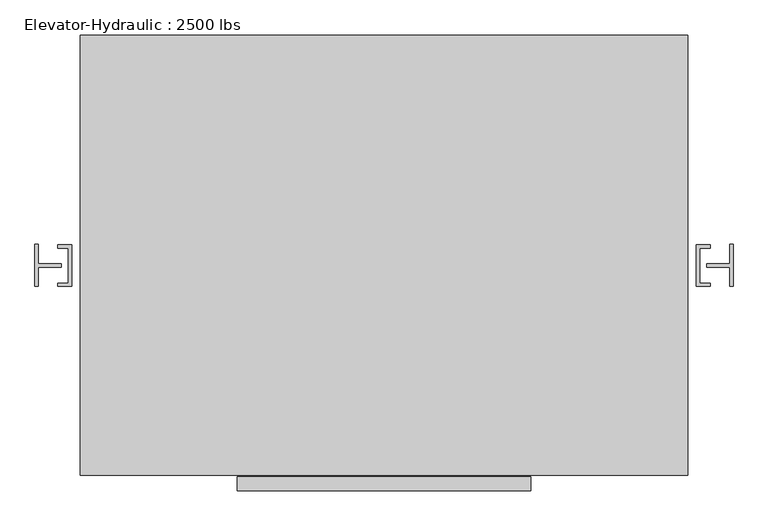
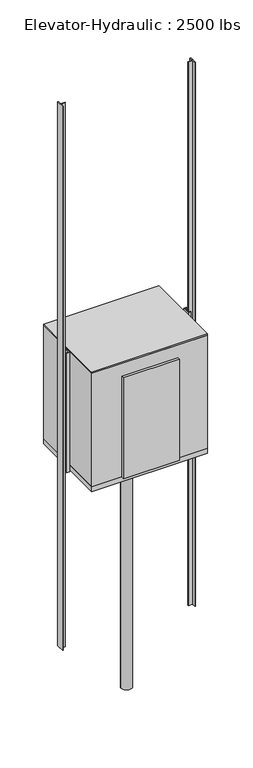
"""IFC4 building model written with IfcOpenShell, lengths in millimetres: proxy geometry, Elevator-Hydraulic : 2500 lbs."""

from ifc_helpers import new_model, si_unit, point, frame, frame_2d, origin, origin_with_axes, place, context, project, spatial, polyline, circle_curve, trimmed, segment, composite_curve, outline, extrude, faceted_brep, source, transform, mapped, element, save


def elevator_hydraulic_2500_lbs_0286828a(model_context):
    return source(origin(), model_context, "Body", "SolidModel", [
        extrude(outline(polyline([(540.8469965, -765.5281737), (540.8469965, -816.3281737), (-525.9530035, -816.3281737), (-525.9530035, -765.5281737), (540.8469965, -765.5281737)])), frame((0.0, 0.0, 3657.6), z_axis=(0.0, 0.0, 1.0), x_axis=(1.0, 0.0, 0.0)), (0.0, 0.0, 1.0), 2032.0),
        extrude(outline(polyline([(1112.3469965, 841.0218263), (1112.3469965, -759.1781737), (-1097.4530035, -759.1781737), (-1097.4530035, 841.0218263), (1112.3469965, 841.0218263)])), frame((0.0, 0.0, 5943.6), z_axis=(0.0, 0.0, 1.0), x_axis=(1.0, 0.0, 0.0)), (0.0, 0.0, 1.0), 25.4),
        extrude(outline(composite_curve([segment(trimmed(circle_curve(frame_2d((7.4469965, 2.8218263)), 101.6), [point((-94.1530035, 2.8218263))], [point((109.0469965, 2.8218263))], False, "CARTESIAN"), True, "CONTINUOUS"), segment(trimmed(circle_curve(frame_2d((7.4469965, 2.8218263)), 101.6), [point((109.0469965, 2.8218263))], [point((-94.1530035, 2.8218263))], False, "CARTESIAN"), True, "CONTINUOUS")], self_intersect=False)), frame((0.0, 0.0, -1219.2), z_axis=(0.0, 0.0, 1.0), x_axis=(1.0, 0.0, 0.0)), (0.0, 0.0, 1.0), 4775.2),
        faceted_brep([(1112.3469965, 841.0218263, 5943.6), (-1097.4530035, 841.0218263, 5943.6), (-1097.4530035, -759.1781737, 5943.6), (1112.3469965, -759.1781737, 5943.6), (1074.2469965, 802.9218263, 5943.6), (1074.2469965, -721.0781737, 5943.6), (-1059.3530035, -721.0781737, 5943.6), (-1059.3530035, 802.9218263, 5943.6), (1074.2469965, 802.9218263, 3657.6), (-1059.3530035, 802.9218263, 3657.6), (-1059.3530035, -721.0781737, 3657.6), (-525.9530035, -721.0781737, 3657.6), (-525.9530035, -759.1781737, 3657.6), (-1097.4530035, -759.1781737, 3657.6), (-1097.4530035, 841.0218263, 3657.6), (1112.3469965, 841.0218263, 3657.6), (1112.3469965, -759.1781737, 3657.6), (540.8469965, -759.1781737, 3657.6), (540.8469965, -721.0781737, 3657.6), (1074.2469965, -721.0781737, 3657.6), (540.8469965, -721.0781737, 5689.6), (-525.9530035, -721.0781737, 5689.6), (-525.9530035, -759.1781737, 5689.6), (540.8469965, -759.1781737, 5689.6)], [[[0, 1, 2, 3], [4, 5, 6, 7]], [[8, 9, 10, 11, 12, 13, 14, 15, 16, 17, 18, 19]], [[5, 4, 8, 19]], [[6, 5, 19, 18, 20, 21, 11, 10]], [[7, 6, 10, 9]], [[4, 7, 9, 8]], [[1, 0, 15, 14]], [[2, 1, 14, 13]], [[3, 2, 13, 12, 22, 23, 17, 16]], [[0, 3, 16, 15]], [[22, 21, 20, 23]], [[21, 22, 12, 11]], [[23, 20, 18, 17]]]),
        extrude(outline(polyline([(1112.3469965, 841.0218263), (1112.3469965, -759.1781737), (-1097.4530035, -759.1781737), (-1097.4530035, 841.0218263), (1112.3469965, 841.0218263)])), frame((0.0, 0.0, 3556.0), z_axis=(0.0, 0.0, 1.0), x_axis=(1.0, 0.0, 0.0)), (0.0, 0.0, 1.0), 101.6),
        extrude(outline(polyline([(-1129.2030035, 79.0218263), (-1129.2030035, -73.3781737), (-1180.0030035, -73.3781737), (-1180.0030035, -60.6781737), (-1141.9030035, -60.6781737), (-1141.9030035, 66.3218263), (-1180.0030035, 66.3218263), (-1180.0030035, 79.0218263), (-1129.2030035, 79.0218263)])), frame((0.0, 0.0, 3556.0), z_axis=(0.0, 0.0, 1.0), x_axis=(1.0, 0.0, 0.0)), (0.0, 0.0, 1.0), 2413.0),
        extrude(outline(polyline([(1144.0969965, 79.0218263), (1194.8969965, 79.0218263), (1194.8969965, 66.3218263), (1156.7969965, 66.3218263), (1156.7969965, -60.6781737), (1194.8969965, -60.6781737), (1194.8969965, -73.3781737), (1144.0969965, -73.3781737), (1144.0969965, 79.0218263)])), frame((0.0, 0.0, 3556.0), z_axis=(0.0, 0.0, 1.0), x_axis=(1.0, 0.0, 0.0)), (0.0, 0.0, 1.0), 2413.0),
        extrude(outline(polyline([(-1249.8530035, 79.0218263), (-1249.8530035, 9.1718263), (-1167.3030035, 9.1718263), (-1167.3030035, -3.5281737), (-1249.8530035, -3.5281737), (-1249.8530035, -73.3781737), (-1262.5530035, -73.3781737), (-1262.5530035, 79.0218263), (-1249.8530035, 79.0218263)])), origin_with_axes(), (0.0, 0.0, 1.0), 10972.8),
        extrude(outline(polyline([(1264.7469965, 79.0218263), (1277.4469965, 79.0218263), (1277.4469965, -73.3781737), (1264.7469965, -73.3781737), (1264.7469965, -3.5281737), (1182.1969965, -3.5281737), (1182.1969965, 9.1718263), (1264.7469965, 9.1718263), (1264.7469965, 79.0218263)])), origin_with_axes(), (0.0, 0.0, 1.0), 10972.8),
    ])


if __name__ == "__main__":
    model = new_model("IFC4")
    model_context = context("Model", 3, world=origin())
    ifc_project = project(units=[si_unit("LENGTHUNIT", "METRE", prefix="MILLI")], contexts=[model_context])
    site = spatial("IfcSite", under=ifc_project)
    building = spatial("IfcBuilding", under=site)
    placement = place(None, origin())
    elevator_hydraulic_2500_lbs_shape = elevator_hydraulic_2500_lbs_0286828a(model_context)
    element("IfcBuildingElementProxy", 1, Name="Elevator-Hydraulic : 2500 lbs", ObjectType="Elevator-Hydraulic : 2500 lbs", at=placement, inside=building, context=model_context, shape_type="MappedRepresentation", body=[
        mapped(elevator_hydraulic_2500_lbs_shape, transform((0.0, 0.0, 0.0), x_axis=(1.0, 0.0, 0.0), y_axis=(0.0, 1.0, 0.0), z_axis=(0.0, 0.0, 1.0))),
    ])
    save(model, "model.ifc")

# Revit data of these elements
# Project information
#   Organization Name = "G3B Press"
#   Organization Description = "Paul F. Aubin Cosulting Services, Inc."
#   Building Name = "Revit Essentials for Architecture"
#   Author = "Paul F. Aubin"
#   Author Website = "https://www.paulaubin.com"
#   Copyright = "Copyright © 2020 Paul F Aubin, all rights reserved"
#   Project Issue Date = "8/1/2020"
#   Project Status = "Design Development"
#   Client Name = "Groups and Links"
#   Project Address = "Enter address here"
#   Project Name = "Hotel"
#   Project Number = "2020.06A"
# Type "Elevator-Hydraulic : 2500 lbs"
#   Cab Location = 12' - 0"
#   Width = 8' - 4"
#   Pit Depth = 4' - 0"
#   Height [instance default] = 36' - 0"
#   Door Opening = 3' - 6"
#   Depth = 5' - 9"
#   Cab Width = 7' - 0"
#   Cab Height = 7' - 6"
#   Cab Depth = 5' - 0"
#   Default Elevation = 0
# Element 1 (IfcBuildingElementProxy, "Elevator-Hydraulic : 2500 lbs")
#   Materials on its faces: "Metal - Steel"
# Materials
#   "Metal - Steel": class "Unassigned", colour RGB 199 199 199, transparency 0, Description = "Steel"
